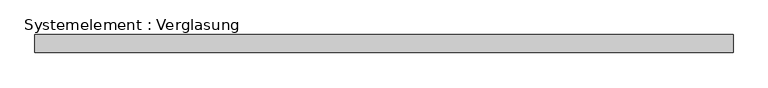
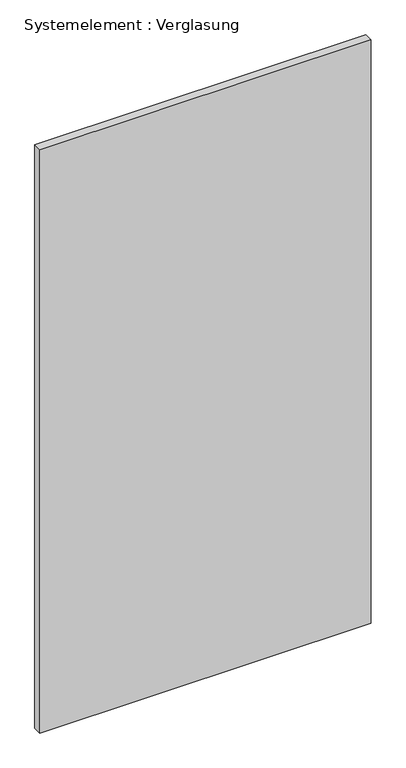
"""IFC4 building model written with IfcOpenShell, lengths in millimetres: plate geometry, Systemelement : Verglasung."""

from ifc_helpers import new_model, si_unit, origin, origin_with_axes, place, context, project, spatial, polyline, outline, extrude, source, transform, mapped, element, save


def systemelement_verglasung_ac3f6550(model_context):
    return source(origin(), model_context, "Body", "SweptSolid", [
        extrude(outline(polyline([(580.0000002, -15.0), (-580.0000002, -15.0), (-580.0000002, 15.0), (580.0000002, 15.0), (580.0000002, -15.0)])), origin_with_axes(), (0.0, 0.0, 1.0), 2160.0),
    ])


if __name__ == "__main__":
    model = new_model("IFC4")
    model_context = context("Model", 3, world=origin())
    ifc_project = project(units=[si_unit("LENGTHUNIT", "METRE", prefix="MILLI")], contexts=[model_context])
    site = spatial("IfcSite", under=ifc_project)
    building = spatial("IfcBuilding", under=site)
    placement = place(None, origin())
    systemelement_verglasung_shape = systemelement_verglasung_ac3f6550(model_context)
    element("IfcPlate", 1, ObjectType="Systemelement : Verglasung", at=placement, inside=building, context=model_context, shape_type="MappedRepresentation", body=[
        mapped(systemelement_verglasung_shape, transform((0.0, 0.0, 0.0), x_axis=(1.0, 0.0, 0.0), y_axis=(0.0, 1.0, 0.0), z_axis=(0.0, 0.0, 1.0))),
    ])
    save(model, "model.ifc")

# Revit data of these elements
# Type "Systemelement : Verglasung"
#   Construction Type Id = "GSP4R"
#   Analytic Construction = "1/8 Zoll Pilkington-Verglasung einfach"
#   Visual Light Transmittance = 0.9
#   Solar Heat Gain Coefficient = 0.86
#   Heat Transfer Coefficient (U) = 6.7069 W/(m²·K)
# Element 1 (IfcPlate, "Systemelement : Verglasung")
#   Materials on its faces: "Glas"
# Materials
#   "Glas": class "Glas", colour RGB 0 0 255, transparency 0.75, Comments = "Render-Darstellung nicht aktualisiert ", Cost = 0
